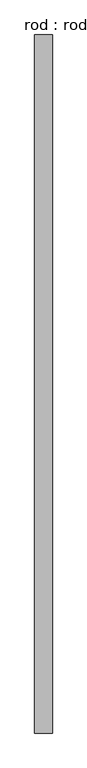
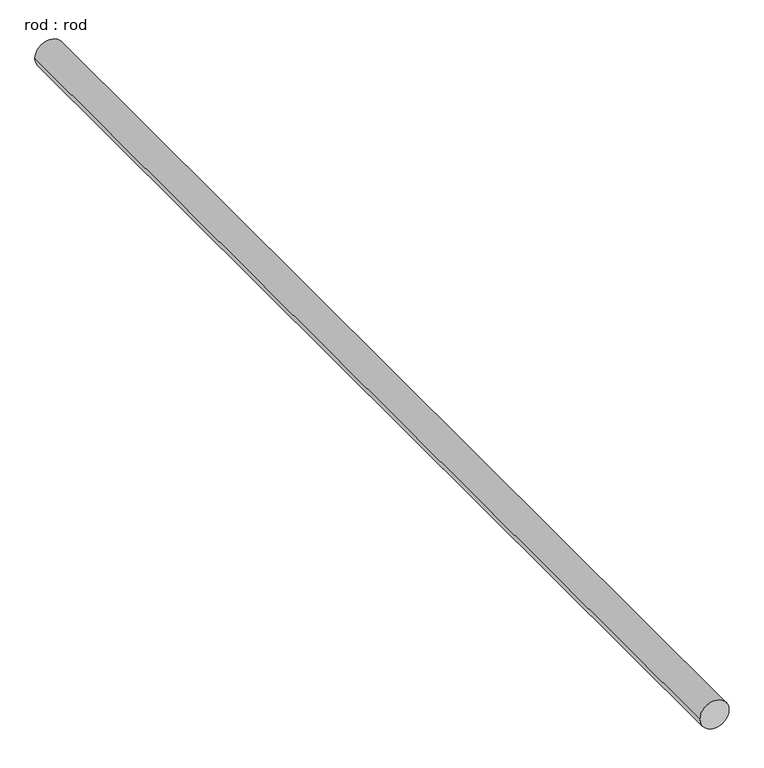
"""IFC4 building model written with IfcOpenShell, lengths in millimetres: proxy geometry, rod : rod."""

from ifc_helpers import new_model, si_unit, point, frame, frame_2d, origin, place, context, project, spatial, circle_curve, trimmed, segment, composite_curve, outline, extrude, source, transform, mapped, element, save


def rod_rod_4d7d1b26(model_context):
    return source(origin(), model_context, "Body", "SweptSolid", [
        extrude(outline(composite_curve([segment(trimmed(circle_curve(frame_2d((0.0108462, 0.0)), 200.0), [point((0.0108462, 200.0))], [point((0.0108462, -200.0))], False, "CARTESIAN"), True, "CONTINUOUS"), segment(trimmed(circle_curve(frame_2d((0.0108462, 0.0)), 200.0), [point((0.0108462, -200.0))], [point((0.0108462, 200.0))], False, "CARTESIAN"), True, "CONTINUOUS")], self_intersect=False)), frame((0.0, -3817.2979213, 0.0), z_axis=(0.0, 1.0, 0.0), x_axis=(0.0, 0.0, 1.0)), (0.0, 0.0, 1.0), 15820.0530733),
    ])


if __name__ == "__main__":
    model = new_model("IFC4")
    model_context = context("Model", 3, world=origin())
    ifc_project = project(units=[si_unit("LENGTHUNIT", "METRE", prefix="MILLI")], contexts=[model_context])
    site = spatial("IfcSite", under=ifc_project)
    building = spatial("IfcBuilding", under=site)
    placement = place(None, origin())
    rod_rod_shape = rod_rod_4d7d1b26(model_context)
    element("IfcBuildingElementProxy", 1, Name="rod : rod", ObjectType="rod : rod", at=placement, inside=building, context=model_context, shape_type="MappedRepresentation", body=[
        mapped(rod_rod_shape, transform((0.0, 0.0, 0.0), x_axis=(1.0, 0.0, 0.0), y_axis=(0.0, 1.0, 0.0), z_axis=(0.0, 0.0, 1.0))),
    ])
    save(model, "model.ifc")

# Revit data of these elements
# Type "rod : rod"
#   Default Elevation = 0
